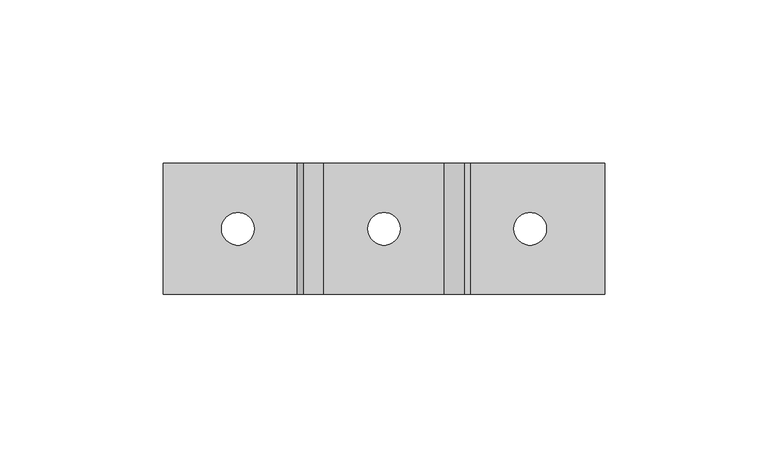
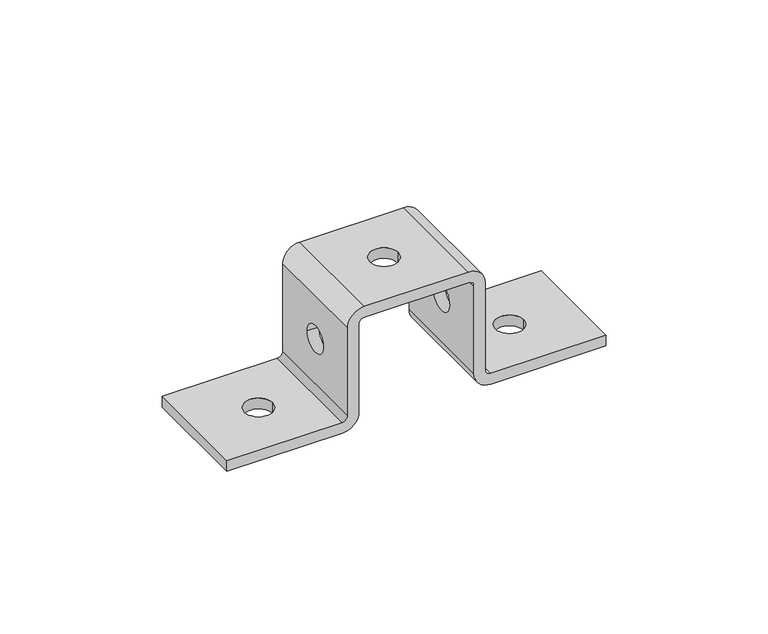
"""IFC4 building model written with IfcOpenShell, lengths in millimetres: proxy geometry, ▶ TN_Скоба соединительная (сборка тип 1) : ▶ TN_Скоба соединительная (сборка тип 1)."""

import ifcopenshell
import ifcopenshell.guid

model = None  # the IFC model being written
_history = None  # IfcOwnerHistory: only IFC2X3 demands one
_inside = {}  # id of a spatial element -> (the spatial element, [elements in it])
_under = {}  # id of a project, library or spatial element -> (it, [spatial elements below it])
_declared = {}  # id of a project -> (the project, [libraries it declares])
_typed = {}  # id of a type object -> (the type object, [elements of that type])
_made_of = {}  # id of a material, layer set ... -> (it, [elements and type objects made of it])


def new_model(schema):
    """Start an empty IFC model of exactly this schema.

    Asked for "IFC4X3", IfcOpenShell would pick the latest addendum, in which some entities
    have other attributes; the version numbers below select the first issue.
    IFC2X3 requires an IfcOwnerHistory on every rooted entity: one is made here for all.
    """
    global model, _history
    if schema == "IFC4X3":
        model = ifcopenshell.file(schema_version=(4, 3, 0, 0))
    else:
        model = ifcopenshell.file(schema=schema)
    _inside.clear()
    _under.clear()
    _declared.clear()
    _typed.clear()
    _made_of.clear()
    _history = None
    if model.schema == "IFC2X3":
        org = make("IfcOrganization", Name="unknown")
        user = make(
            "IfcPersonAndOrganization",
            ThePerson=make("IfcPerson", FamilyName="unknown"),
            TheOrganization=org,
        )
        app = make(
            "IfcApplication",
            ApplicationDeveloper=org,
            Version="unknown",
            ApplicationFullName="unknown",
            ApplicationIdentifier="unknown",
        )
        _history = make(
            "IfcOwnerHistory",
            OwningUser=user,
            OwningApplication=app,
            ChangeAction="ADDED",
            CreationDate=0,
        )
    return model


def make(cls, **values):
    """One entity of the class cls with the attributes given. An attribute that is None is left unset."""
    return model.create_entity(
        cls, **{name: value for name, value in values.items() if value is not None}
    )


def rooted(cls, **values):
    """An entity with a GlobalId (a new one), such as an element, a storey or a relation."""
    return make(cls, GlobalId=ifcopenshell.guid.new(), OwnerHistory=_history, **values)


def si_unit(unit_type, name, prefix=None):
    """IfcSIUnit, for example si_unit("LENGTHUNIT", "METRE", prefix="MILLI")."""
    return make("IfcSIUnit", UnitType=unit_type, Prefix=prefix, Name=name)


def assignment(units):
    """IfcUnitAssignment: the units of a project."""
    return None if units is None else make("IfcUnitAssignment", Units=units)


def point(xyz):
    """IfcCartesianPoint."""
    return None if xyz is None else make("IfcCartesianPoint", Coordinates=xyz)


def direction(xyz):
    """IfcDirection."""
    return None if xyz is None else make("IfcDirection", DirectionRatios=xyz)


def frame(location, z_axis=None, x_axis=None):
    """IfcAxis2Placement3D, a coordinate frame: its origin and axes. An axis left out is left unset."""
    return make(
        "IfcAxis2Placement3D",
        Location=point(location),
        Axis=direction(z_axis),
        RefDirection=direction(x_axis),
    )


def origin():
    """The frame at (0, 0, 0) with its axes left unset."""
    return frame((0.0, 0.0, 0.0))


def place(relative_to, where):
    """IfcLocalPlacement: puts the frame where relative to a parent placement (None: the world)."""
    return make(
        "IfcLocalPlacement", PlacementRelTo=relative_to, RelativePlacement=where
    )


def context(
    kind, dimensions, precision=None, world=None, true_north=None, identifier=None
):
    """IfcGeometricRepresentationContext, for example the 3D "Model" context."""
    return make(
        "IfcGeometricRepresentationContext",
        ContextIdentifier=identifier,
        ContextType=kind,
        CoordinateSpaceDimension=dimensions,
        Precision=precision,
        WorldCoordinateSystem=world,
        TrueNorth=true_north,
    )


def project(units=None, contexts=None):
    """IfcProject with its units and contexts."""
    return rooted(
        "IfcProject",
        Name="project",
        RepresentationContexts=contexts,
        UnitsInContext=assignment(units),
    )


def spatial(cls, under=None, at=None, **own):
    """A site, building, storey or space (cls), placed at a placement, below another one or the project."""
    s = rooted(cls, ObjectPlacement=at, **own)
    if under is not None:
        _under.setdefault(under.id(), (under, []))[1].append(s)
    return s


def polyline(points):
    """IfcPolyline through the points."""
    return make("IfcPolyline", Points=[point(p) for p in points])


def circle_curve(where, radius):
    """IfcCircle in the frame where."""
    return make("IfcCircle", Position=where, Radius=radius)


def shape(context_of_items, identifier, shape_type, items):
    """IfcShapeRepresentation: the items that make up one representation, for example the "Body"."""
    return make(
        "IfcShapeRepresentation",
        ContextOfItems=context_of_items,
        RepresentationIdentifier=identifier,
        RepresentationType=shape_type,
        Items=items,
    )


def source(mapping_origin, context_of_items, identifier, shape_type, items):
    """IfcRepresentationMap: a shape defined once, which mapped items show again and again."""
    return make(
        "IfcRepresentationMap",
        MappingOrigin=mapping_origin,
        MappedRepresentation=shape(context_of_items, identifier, shape_type, items),
    )


def transform(
    local_origin,
    x_axis=None,
    y_axis=None,
    z_axis=None,
    scale=None,
    scale2=None,
    scale3=None,
    uniform=True,
):
    """IfcCartesianTransformationOperator3D, or its non-uniform kind. x_axis, y_axis, z_axis: its Axis1, 2, 3."""
    if uniform:
        return make(
            "IfcCartesianTransformationOperator3D",
            Axis1=direction(x_axis),
            Axis2=direction(y_axis),
            LocalOrigin=point(local_origin),
            Scale=scale,
            Axis3=direction(z_axis),
        )
    return make(
        "IfcCartesianTransformationOperator3DnonUniform",
        Axis1=direction(x_axis),
        Axis2=direction(y_axis),
        LocalOrigin=point(local_origin),
        Scale=scale,
        Axis3=direction(z_axis),
        Scale2=scale2,
        Scale3=scale3,
    )


def mapped(mapping_source, mapping_target):
    """IfcMappedItem: shows the shape of a source again, moved by a transform."""
    return make(
        "IfcMappedItem", MappingSource=mapping_source, MappingTarget=mapping_target
    )


def made_of(thing, what):
    """Note that an element or type object is made of a material, layer set ...; save() writes the relation."""
    if what is not None:
        _made_of.setdefault(what.id(), (what, []))[1].append(thing)
    return thing


def element(
    cls,
    number,
    at=None,
    inside=None,
    cuts=None,
    type_object=None,
    material=None,
    context=None,
    identifier="Body",
    shape_type=None,
    held_by="IfcProductDefinitionShape",
    body=None,
    shapes=None,
    **own,
):
    """One element of the class cls, such as IfcWall. Its Tag is "e" and its number.

    at: its placement. inside: the storey or other place that contains it. cuts: it is an
    opening in that element (IfcRelVoidsElement). A single representation is given by context,
    identifier, shape_type and body (its items); several are given by shapes. held_by: the class
    of the entity that holds the representations. save() writes the other relations.
    """
    e = rooted(cls, Tag="e%d" % number, ObjectPlacement=at, **own)
    if body is not None:
        shapes = [shape(context, identifier, shape_type, body)]
    if shapes is not None:
        e.Representation = make(held_by, Representations=shapes)
    if inside is not None:
        _inside.setdefault(inside.id(), (inside, []))[1].append(e)
    if cuts is not None:
        rooted(
            "IfcRelVoidsElement", RelatingBuildingElement=cuts, RelatedOpeningElement=e
        )
    if type_object is not None:
        _typed.setdefault(type_object.id(), (type_object, []))[1].append(e)
    return made_of(e, material)


def aggregate(whole, parts):
    """IfcRelAggregates: a whole, such as a stair, and the parts it consists of."""
    return rooted("IfcRelAggregates", RelatingObject=whole, RelatedObjects=parts)


def save(model, path):
    """Write the relations noted so far, then the file.

    IfcRelAggregates (storeys below a building ...), IfcRelContainedInSpatialStructure (elements
    in a storey), IfcRelDefinesByType, IfcRelAssociatesMaterial and IfcRelDeclares: one each for
    every whole, place, type object, material and project.
    """
    for whole, parts in _under.values():
        aggregate(whole, parts)
    for where, things in _inside.values():
        rooted(
            "IfcRelContainedInSpatialStructure",
            RelatedElements=things,
            RelatingStructure=where,
        )
    for kind, things in _typed.values():
        rooted("IfcRelDefinesByType", RelatedObjects=things, RelatingType=kind)
    for what, things in _made_of.values():
        rooted("IfcRelAssociatesMaterial", RelatedObjects=things, RelatingMaterial=what)
    for by, libraries in _declared.values():
        rooted("IfcRelDeclares", RelatingContext=by, RelatedDefinitions=libraries)
    model.write(path)


def plane_surface(at):
    """IfcPlane: the flat surface through the origin of the frame at, square to its z axis."""
    return make("IfcPlane", Position=at)


def cylinder_surface(at, radius):
    """IfcCylindricalSurface: all points at the distance radius from the z axis of the frame at."""
    return make("IfcCylindricalSurface", Position=at, Radius=radius)


def revolved_surface(curve, axis_point, axis_direction):
    """IfcSurfaceOfRevolution: the curve turned about the line through axis_point along axis_direction."""
    return make(
        "IfcSurfaceOfRevolution",
        SweptCurve=make("IfcArbitraryOpenProfileDef", ProfileType="CURVE", Curve=curve),
        AxisPosition=make("IfcAxis1Placement", Location=point(axis_point), Axis=direction(axis_direction)),
    )


def advanced_brep(points, edges, surfaces, faces):
    """IfcAdvancedBrep: a solid bounded by faces that lie on surfaces and meet in shared edges.

    An edge is (start, end): straight between two places in points (the first is 0);
    or (start, end, curve); or (start, end, curve, False) where it runs against its curve.
    A face is (place in surfaces, loops), or (place, loops, False) where it looks against
    its surface's normal. A loop lists edges by number (the first is 1), with a minus sign
    where the edge is run from its end to its start. The first loop is the outer one.
    """
    corners = [point(p) for p in points]
    vertices = [make("IfcVertexPoint", VertexGeometry=c) for c in corners]
    made = []
    for start, end, *more in edges:
        made.append(
            make(
                "IfcEdgeCurve",
                EdgeStart=vertices[start],
                EdgeEnd=vertices[end],
                EdgeGeometry=more[0] if more else make("IfcPolyline", Points=[corners[start], corners[end]]),
                SameSense=more[1] if len(more) > 1 else True,
            )
        )
    hull = []
    for where, loops, *sense in faces:
        bounds = []
        for j, loop in enumerate(loops):
            ring = [make("IfcOrientedEdge", EdgeElement=made[abs(k) - 1], Orientation=k > 0) for k in loop]
            bounds.append(
                make(
                    "IfcFaceOuterBound" if j == 0 else "IfcFaceBound",
                    Bound=make("IfcEdgeLoop", EdgeList=ring),
                    Orientation=True,
                )
            )
        hull.append(make("IfcAdvancedFace", Bounds=bounds, FaceSurface=surfaces[where], SameSense=sense[0] if sense else True))
    return make("IfcAdvancedBrep", Outer=make("IfcClosedShell", CfsFaces=hull))


def generic_models_910e0f76(model_context):
    return source(origin(), model_context, "Body", "AdvancedBrep", [
        advanced_brep(
        [(-26.5, -20.0, 0.0), (-20.5, -20.0, 6.0), (-20.5, -20.0, 39.0), (-18.5, -20.0, 41.0), (18.5, -20.0, 41.0), (20.5, -20.0, 39.0), (20.5, -20.0, 6.0), (26.5, -20.0, 0.0), (67.5, -20.0, 0.0), (67.5, -20.0, 4.0), (26.5, -20.0, 4.0), (24.5, -20.0, 6.0), (24.5, -20.0, 39.0), (18.5, -20.0, 45.0), (-18.5, -20.0, 45.0), (-24.5, -20.0, 39.0), (-24.5, -20.0, 6.0), (-26.5, -20.0, 4.0), (-67.5, -20.0, 4.0), (-67.5, -20.0, 0.0), (-26.5, 20.0, 0.0), (-67.5, 20.0, 0.0), (-67.5, 20.0, 4.0), (-26.5, 20.0, 4.0), (-24.5, 20.0, 6.0), (-24.5, 20.0, 39.0), (-18.5, 20.0, 45.0), (18.5, 20.0, 45.0), (24.5, 20.0, 39.0), (24.5, 20.0, 6.0), (26.5, 20.0, 4.0), (67.5, 20.0, 4.0), (67.5, 20.0, 0.0), (26.5, 20.0, 0.0), (20.5, 20.0, 6.0), (20.5, 20.0, 39.0), (18.5, 20.0, 41.0), (-18.5, 20.0, 41.0), (-20.5, 20.0, 39.0), (-20.5, 20.0, 6.0), (-20.5, 5.0, 22.7939035), (-20.5, -5.0, 22.7939035), (-5.0, 0.0, 41.0), (5.0, 0.0, 41.0), (20.5, -5.0, 22.7939035), (20.5, 5.0, 22.7939035), (39.7162685, 0.0, 0.0), (49.7162685, 0.0, 0.0), (49.7162685, 0.0, 4.0), (39.7162685, 0.0, 4.0), (24.5, 5.0, 22.7939035), (24.5, -5.0, 22.7939035), (5.0, 0.0, 45.0), (-5.0, 0.0, 45.0), (-24.5, -5.0, 22.7939035), (-24.5, 5.0, 22.7939035), (-39.7162685, 0.0, 4.0), (-49.7162685, 0.0, 4.0), (-49.7162685, 0.0, 0.0), (-39.7162685, 0.0, 0.0)],
        [
            (0, 1, circle_curve(frame((-26.5, -20.0, 6.0), z_axis=(0.0, -1.0, 0.0), x_axis=(0.0, 0.0, -1.0)), 6.0)),
            (1, 2),
            (2, 3, circle_curve(frame((-18.5, -20.0, 39.0), z_axis=(0.0, 1.0, 0.0), x_axis=(0.0, 0.0, -1.0)), 2.0)),
            (3, 4),
            (4, 5, circle_curve(frame((18.5, -20.0, 39.0), z_axis=(0.0, 1.0, 0.0), x_axis=(0.0, 0.0, -1.0)), 2.0)),
            (5, 6),
            (6, 7, circle_curve(frame((26.5, -20.0, 6.0), z_axis=(0.0, -1.0, 0.0), x_axis=(0.0, 0.0, -1.0)), 6.0)),
            (7, 8),
            (8, 9),
            (9, 10),
            (10, 11, circle_curve(frame((26.5, -20.0, 6.0), z_axis=(0.0, 1.0, 0.0), x_axis=(0.0, 0.0, -1.0)), 2.0)),
            (11, 12),
            (12, 13, circle_curve(frame((18.5, -20.0, 39.0), z_axis=(0.0, -1.0, 0.0), x_axis=(0.0, 0.0, -1.0)), 6.0)),
            (13, 14),
            (14, 15, circle_curve(frame((-18.5, -20.0, 39.0), z_axis=(0.0, -1.0, 0.0), x_axis=(0.0, 0.0, -1.0)), 6.0)),
            (15, 16),
            (16, 17, circle_curve(frame((-26.5, -20.0, 6.0), z_axis=(0.0, 1.0, 0.0), x_axis=(0.0, 0.0, -1.0)), 2.0)),
            (17, 18),
            (18, 19),
            (19, 0),
            (20, 21),
            (21, 22),
            (22, 23),
            (23, 24, circle_curve(frame((-26.5, 20.0, 6.0), z_axis=(0.0, -1.0, 0.0), x_axis=(0.0, 0.0, -1.0)), 2.0)),
            (24, 25),
            (25, 26, circle_curve(frame((-18.5, 20.0, 39.0), z_axis=(0.0, 1.0, 0.0), x_axis=(0.0, 0.0, -1.0)), 6.0)),
            (26, 27),
            (27, 28, circle_curve(frame((18.5, 20.0, 39.0), z_axis=(0.0, 1.0, 0.0), x_axis=(0.0, 0.0, -1.0)), 6.0)),
            (28, 29),
            (29, 30, circle_curve(frame((26.5, 20.0, 6.0), z_axis=(0.0, -1.0, 0.0), x_axis=(0.0, 0.0, -1.0)), 2.0)),
            (30, 31),
            (31, 32),
            (32, 33),
            (33, 34, circle_curve(frame((26.5, 20.0, 6.0), z_axis=(0.0, 1.0, 0.0), x_axis=(0.0, 0.0, -1.0)), 6.0)),
            (34, 35),
            (35, 36, circle_curve(frame((18.5, 20.0, 39.0), z_axis=(0.0, -1.0, 0.0), x_axis=(0.0, 0.0, -1.0)), 2.0)),
            (36, 37),
            (37, 38, circle_curve(frame((-18.5, 20.0, 39.0), z_axis=(0.0, -1.0, 0.0), x_axis=(0.0, 0.0, -1.0)), 2.0)),
            (38, 39),
            (39, 20, circle_curve(frame((-26.5, 20.0, 6.0), z_axis=(0.0, 1.0, 0.0), x_axis=(0.0, 0.0, -1.0)), 6.0)),
            (0, 20),
            (39, 1),
            (38, 2),
            (40, 41, circle_curve(frame((-20.5, 0.0, 22.7939035), z_axis=(-1.0, 0.0, 0.0), x_axis=(0.0, 1.0, 0.0)), 5.0)),
            (41, 40, circle_curve(frame((-20.5, 0.0, 22.7939035), z_axis=(-1.0, 0.0, 0.0), x_axis=(0.0, 1.0, 0.0)), 5.0)),
            (37, 3),
            (36, 4),
            (42, 43, circle_curve(frame((0.0, 0.0, 41.0), z_axis=(0.0, 0.0, 1.0), x_axis=(1.0, 0.0, 0.0)), 5.0)),
            (43, 42, circle_curve(frame((0.0, 0.0, 41.0), z_axis=(0.0, 0.0, 1.0), x_axis=(1.0, 0.0, 0.0)), 5.0)),
            (35, 5),
            (34, 6),
            (44, 45, circle_curve(frame((20.5, 0.0, 22.7939035), z_axis=(1.0, 0.0, 0.0), x_axis=(0.0, 1.0, 0.0)), 5.0)),
            (45, 44, circle_curve(frame((20.5, 0.0, 22.7939035), z_axis=(1.0, 0.0, 0.0), x_axis=(0.0, 1.0, 0.0)), 5.0)),
            (33, 7),
            (32, 8),
            (46, 47, circle_curve(frame((44.7162685, 0.0, 0.0), z_axis=(0.0, 0.0, 1.0), x_axis=(1.0, 0.0, 0.0)), 5.0)),
            (47, 46, circle_curve(frame((44.7162685, 0.0, 0.0), z_axis=(0.0, 0.0, 1.0), x_axis=(1.0, 0.0, 0.0)), 5.0)),
            (31, 9),
            (30, 10),
            (48, 49, circle_curve(frame((44.7162685, 0.0, 4.0), z_axis=(0.0, 0.0, -1.0), x_axis=(1.0, 0.0, 0.0)), 5.0)),
            (49, 48, circle_curve(frame((44.7162685, 0.0, 4.0), z_axis=(0.0, 0.0, -1.0), x_axis=(1.0, 0.0, 0.0)), 5.0)),
            (29, 11),
            (28, 12),
            (50, 51, circle_curve(frame((24.5, 0.0, 22.7939035), z_axis=(-1.0, 0.0, 0.0), x_axis=(0.0, 1.0, 0.0)), 5.0)),
            (51, 50, circle_curve(frame((24.5, 0.0, 22.7939035), z_axis=(-1.0, 0.0, 0.0), x_axis=(0.0, 1.0, 0.0)), 5.0)),
            (27, 13),
            (26, 14),
            (52, 53, circle_curve(frame((0.0, 0.0, 45.0), z_axis=(0.0, 0.0, -1.0), x_axis=(1.0, 0.0, 0.0)), 5.0)),
            (53, 52, circle_curve(frame((0.0, 0.0, 45.0), z_axis=(0.0, 0.0, -1.0), x_axis=(1.0, 0.0, 0.0)), 5.0)),
            (25, 15),
            (24, 16),
            (54, 55, circle_curve(frame((-24.5, 0.0, 22.7939035), z_axis=(1.0, 0.0, 0.0), x_axis=(0.0, 1.0, 0.0)), 5.0)),
            (55, 54, circle_curve(frame((-24.5, 0.0, 22.7939035), z_axis=(1.0, 0.0, 0.0), x_axis=(0.0, 1.0, 0.0)), 5.0)),
            (23, 17),
            (22, 18),
            (56, 57, circle_curve(frame((-44.7162685, 0.0, 4.0), z_axis=(0.0, 0.0, -1.0), x_axis=(1.0, 0.0, 0.0)), 5.0)),
            (57, 56, circle_curve(frame((-44.7162685, 0.0, 4.0), z_axis=(0.0, 0.0, -1.0), x_axis=(1.0, 0.0, 0.0)), 5.0)),
            (21, 19),
            (58, 59, circle_curve(frame((-44.7162685, 0.0, 0.0), z_axis=(0.0, 0.0, 1.0), x_axis=(1.0, 0.0, 0.0)), 5.0)),
            (59, 58, circle_curve(frame((-44.7162685, 0.0, 0.0), z_axis=(0.0, 0.0, 1.0), x_axis=(1.0, 0.0, 0.0)), 5.0)),
            (56, 59),
            (58, 57),
            (48, 47),
            (46, 49),
            (42, 53),
            (52, 43),
            (44, 51),
            (50, 45),
            (54, 41),
            (40, 55),
        ],
        [
            plane_surface(frame((0.0, -20.0, 0.0), z_axis=(0.0, -1.0, 0.0), x_axis=(0.0, 0.0, 1.0))),
            plane_surface(frame((0.0, 20.0, 0.0), z_axis=(0.0, 1.0, 0.0), x_axis=(0.0, 0.0, 1.0))),
            cylinder_surface(frame((-26.5, -20.0, 6.0), z_axis=(0.0, -1.0, 0.0), x_axis=(0.0, 0.0, -1.0)), 6.0),
            plane_surface(frame((-20.5, -20.0, 6.0), z_axis=(1.0, 0.0, 0.0), x_axis=(0.0, 1.0, 0.0))),
            revolved_surface(polyline([(-18.5, 20.0, 37.0), (-18.5, -20.0, 37.0)]), (-18.5, -20.0, 39.0), (0.0, 1.0, 0.0)),
            plane_surface(frame((-18.5, -20.0, 41.0), z_axis=(0.0, 0.0, -1.0), x_axis=(0.0, 1.0, 0.0))),
            revolved_surface(polyline([(18.5, 20.0, 37.0), (18.5, -20.0, 37.0)]), (18.5, -20.0, 39.0), (0.0, 1.0, 0.0)),
            plane_surface(frame((20.5, -20.0, 39.0), z_axis=(-1.0, 0.0, 0.0), x_axis=(0.0, 1.0, 0.0))),
            cylinder_surface(frame((26.5, -20.0, 6.0), z_axis=(0.0, -1.0, 0.0), x_axis=(0.0, 0.0, -1.0)), 6.0),
            plane_surface(frame((26.5, -20.0, 0.0), z_axis=(0.0, 0.0, -1.0), x_axis=(0.0, 1.0, 0.0))),
            plane_surface(frame((67.5, -20.0, 0.0), z_axis=(1.0, 0.0, 0.0), x_axis=(0.0, 1.0, 0.0))),
            plane_surface(frame((67.5, -20.0, 4.0), z_axis=(0.0, 0.0, 1.0), x_axis=(0.0, 1.0, 0.0))),
            revolved_surface(polyline([(26.5, 20.0, 4.0), (26.5, -20.0, 4.0)]), (26.5, -20.0, 6.0), (0.0, 1.0, 0.0)),
            plane_surface(frame((24.5, -20.0, 6.0), z_axis=(1.0, 0.0, 0.0), x_axis=(0.0, 1.0, 0.0))),
            cylinder_surface(frame((18.5, -20.0, 39.0), z_axis=(0.0, -1.0, 0.0), x_axis=(0.0, 0.0, -1.0)), 6.0),
            plane_surface(frame((18.5, -20.0, 45.0), z_axis=(0.0, 0.0, 1.0), x_axis=(0.0, 1.0, 0.0))),
            cylinder_surface(frame((-18.5, -20.0, 39.0), z_axis=(0.0, -1.0, 0.0), x_axis=(0.0, 0.0, -1.0)), 6.0),
            plane_surface(frame((-24.5, -20.0, 39.0), z_axis=(-1.0, 0.0, 0.0), x_axis=(0.0, 1.0, 0.0))),
            revolved_surface(polyline([(-26.5, 20.0, 4.0), (-26.5, -20.0, 4.0)]), (-26.5, -20.0, 6.0), (0.0, 1.0, 0.0)),
            plane_surface(frame((-26.5, -20.0, 4.0), z_axis=(0.0, 0.0, 1.0), x_axis=(0.0, 1.0, 0.0))),
            plane_surface(frame((-67.5, -20.0, 4.0), z_axis=(-1.0, 0.0, 0.0), x_axis=(0.0, 1.0, 0.0))),
            plane_surface(frame((-67.5, -20.0, 0.0), z_axis=(0.0, 0.0, -1.0), x_axis=(0.0, 1.0, 0.0))),
            revolved_surface(polyline([(-39.7162685, 0.0, 4.0), (-39.7162685, 0.0, 0.0)]), (-44.7162685, 0.0, 0.0), (0.0, 0.0, 1.0)),
            revolved_surface(polyline([(49.7162685, 0.0, 4.0), (49.7162685, 0.0, 0.0)]), (44.7162685, 0.0, 0.0), (0.0, 0.0, 1.0)),
            revolved_surface(polyline([(5.0, 0.0, 45.0), (5.0, 0.0, 41.0)]), (0.0, 0.0, 35.2036226), (0.0, 0.0, 1.0)),
            revolved_surface(polyline([(24.5, 5.0, 22.7939035), (20.5, 5.0, 22.7939035)]), (-39.393858, 0.0, 22.7939035), (1.0, 0.0, 0.0)),
            revolved_surface(polyline([(-20.5, 5.0, 22.7939035), (-24.5, 5.0, 22.7939035)]), (-39.393858, 0.0, 22.7939035), (1.0, 0.0, 0.0)),
        ],
        [
            (0, [[1, 2, 3, 4, 5, 6, 7, 8, 9, 10, 11, 12, 13, 14, 15, 16, 17, 18, 19, 20]]),
            (1, [[21, 22, 23, 24, 25, 26, 27, 28, 29, 30, 31, 32, 33, 34, 35, 36, 37, 38, 39, 40]]),
            (2, [[-1, 41, -40, 42]]),
            (3, [[-2, -42, -39, 43], [44, 45]]),
            (4, [[-3, -43, -38, 46]]),
            (5, [[-4, -46, -37, 47], [48, 49]]),
            (6, [[-5, -47, -36, 50]]),
            (7, [[-6, -50, -35, 51], [52, 53]]),
            (8, [[-7, -51, -34, 54]]),
            (9, [[-8, -54, -33, 55], [56, 57]]),
            (10, [[-9, -55, -32, 58]]),
            (11, [[-10, -58, -31, 59], [60, 61]]),
            (12, [[-11, -59, -30, 62]]),
            (13, [[-12, -62, -29, 63], [64, 65]]),
            (14, [[-13, -63, -28, 66]]),
            (15, [[-14, -66, -27, 67], [68, 69]]),
            (16, [[-15, -67, -26, 70]]),
            (17, [[-16, -70, -25, 71], [72, 73]]),
            (18, [[-17, -71, -24, 74]]),
            (19, [[-18, -74, -23, 75], [76, 77]]),
            (20, [[-19, -75, -22, 78]]),
            (21, [[-20, -78, -21, -41], [79, 80]]),
            (22, [[81, -79, 82, -76]]),
            (22, [[-81, -77, -82, -80]]),
            (23, [[83, -56, 84, -60]]),
            (23, [[-83, -61, -84, -57]]),
            (24, [[85, -68, 86, -48]]),
            (24, [[-85, -49, -86, -69]]),
            (25, [[87, -64, 88, -52]]),
            (26, [[89, -44, 90, -72]]),
            (25, [[-87, -53, -88, -65]]),
            (26, [[-89, -73, -90, -45]]),
        ],
    ),
    ])


if __name__ == "__main__":
    model = new_model("IFC4")
    model_context = context("Model", 3, world=origin())
    ifc_project = project(units=[si_unit("LENGTHUNIT", "METRE", prefix="MILLI")], contexts=[model_context])
    site = spatial("IfcSite", under=ifc_project)
    building = spatial("IfcBuilding", under=site)
    placement = place(None, origin())
    generic_models_shape = generic_models_910e0f76(model_context)
    element("IfcBuildingElementProxy", 1, Name="▶ TN_Скоба соединительная (сборка тип 1) : ▶ TN_Скоба соединительная (сборка тип 1)", ObjectType="▶ TN_Скоба соединительная (сборка тип 1) : ▶ TN_Скоба соединительная (сборка тип 1)", at=placement, inside=building, context=model_context, shape_type="MappedRepresentation", body=[
        mapped(generic_models_shape, transform((0.0, 0.0, 0.0), x_axis=(1.0, 0.0, 0.0), y_axis=(0.0, 1.0, 0.0), z_axis=(0.0, 0.0, 1.0))),
    ])
    save(model, "model.ifc")

# Revit data of these elements
# Type "▶ TN_Скоба соединительная (сборка тип 1) : ▶ TN_Скоба соединительная (сборка тип 1)"
#   Description = "Cоединительный элемент для монтажа рам, стеллажей, каркасов для легких и средних систем. Обеспечивает устойчивое поперечное (крестовое) соединение профилей. Наиболее эффективно использования скобы, как соединителя для создания пространственных силовых, опорных каркасов и решеток. Возможность реализации крепления профиля к бетонному основанию."
#   Manufacturer = "ТехноНИКОЛЬ"
#   Model = "Комплектующие к опорам"
#   URL = "https://nav.tn.ru/knowledge-base/polimernye-membrany/opory-pod-oborudovanie-na-ploskoy-krovle/?sphrase_id=266812"
#   ADSK_Обозначение = "ТехноНИКОЛЬ"
#   ADSK_Наименование краткое [instance default] = "С41х124 4F3"
#   ADSK_Наименование [instance default] = "Скоба соединительная 41х124 4F3"
#   ADSK_Масса_Текст = ""
#   ADSK_Марка [instance default] = "С41х124 4F3"
#   ADSK_Код изделия [instance default] = "690885"
#   ADSK_Завод-изготовитель = "ТехноНИКОЛЬ"
#   ADSK_Единица измерения = "шт."
#   ADSK_Группирование = "Комплектующие к опорам"
#   ADSK_URL страницы изделия = "https://nav.tn.ru/knowledge-base/polimernye-membrany/opory-pod-oborudovanie-na-ploskoy-krovle/?sphrase_id=266812"
#   ADSK_URL документации изделия = ""
#   Высота крепежа [instance default] = 84 mm
#   ADSK_Количество = 1
#   Скоба соединительная 41х62 4F3 [instance default] = no
#   Скоба соединительная 41х41 4F5 [instance default] = no
#   Скоба соединительная 41х124 4F3 [instance default] = yes
#   ADSK_Материал = TN_СтальГальванизированная_Серый
#   Default Elevation = 0
# Element 1 (IfcBuildingElementProxy, "▶ TN_Скоба соединительная (сборка тип 1) : ▶ TN_Скоба соединительная (сборка тип 1)")
#   ADSK_Наименование краткое = "С41х41 4F5"
#   ADSK_Наименование = "Скоба соединительная 41х41 4F5"
#   ADSK_Марка = "С41х41 4F5"
#   ADSK_Код изделия = "660818"
#   Высота крепежа = 1 mm
#   Скоба соединительная 41х41 4F5 = yes
#   Скоба соединительная 41х124 4F3 = no
#   Materials on its faces: "TN_СтальГальванизированная_Серый"
# Materials
#   "TN_СтальГальванизированная_Серый": class "Типовые", colour RGB 206 210 213, transparency 0, Cost = 0
